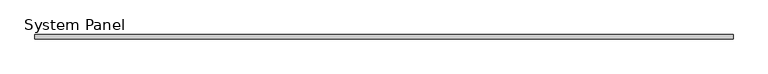
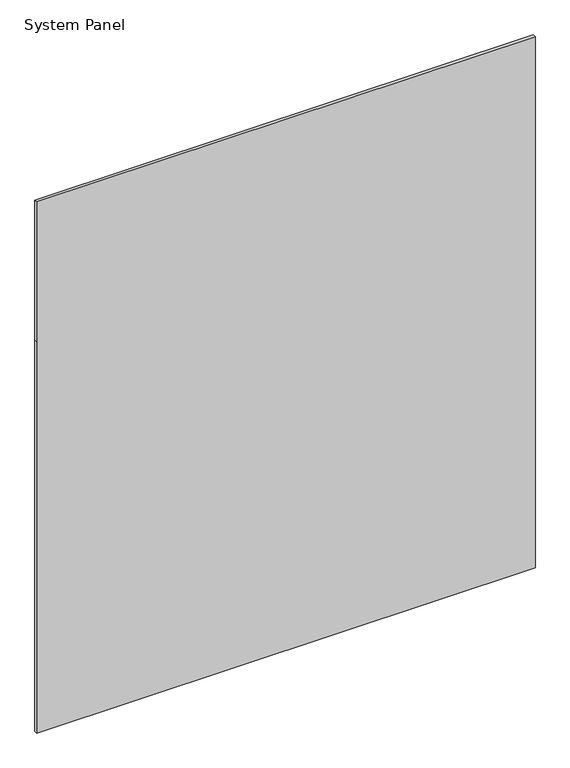
"""IFC4 building model written with IfcOpenShell, lengths in millimetres: plate geometry, System Panel : 로이복층유리_16."""

from ifc_helpers import new_model, si_unit, frame, origin, place, context, project, spatial, polyline, outline, extrude, source, transform, mapped, element, save


def system_panel_2a2c7901(model_context):
    return source(origin(), model_context, "Body", "SweptSolid", [
        extrude(outline(polyline([(0.0, -1312.5), (0.0, 1312.5), (2177.5, 1312.5), (2955.0, 1312.5), (2955.0, -1312.5), (2177.5, -1312.5), (0.0, -1312.5)])), frame((0.0, -8.0, 0.0), z_axis=(0.0, 1.0, 0.0), x_axis=(0.0, 0.0, 1.0)), (0.0, 0.0, 1.0), 16.0),
    ])


if __name__ == "__main__":
    model = new_model("IFC4")
    model_context = context("Model", 3, world=origin())
    ifc_project = project(units=[si_unit("LENGTHUNIT", "METRE", prefix="MILLI")], contexts=[model_context])
    site = spatial("IfcSite", under=ifc_project)
    building = spatial("IfcBuilding", under=site)
    placement = place(None, origin())
    system_panel_shape = system_panel_2a2c7901(model_context)
    element("IfcPlate", 1, ObjectType="System Panel : 로이복층유리_16", at=placement, inside=building, context=model_context, shape_type="MappedRepresentation", body=[
        mapped(system_panel_shape, transform((0.0, 0.0, 0.0), x_axis=(1.0, 0.0, 0.0), y_axis=(0.0, 1.0, 0.0), z_axis=(0.0, 0.0, 1.0))),
    ])
    save(model, "model.ifc")

# Revit data of these elements
# Element 1 (IfcPlate, "System Panel : 로이복층유리_16")
#   Materials on its faces: "00_Glass_Glass"
# Materials
#   "00_Glass_Glass": class "Glass", colour RGB 218 227 224, transparency 0.85, Description = "Glass", Cost = 0, Image = none
